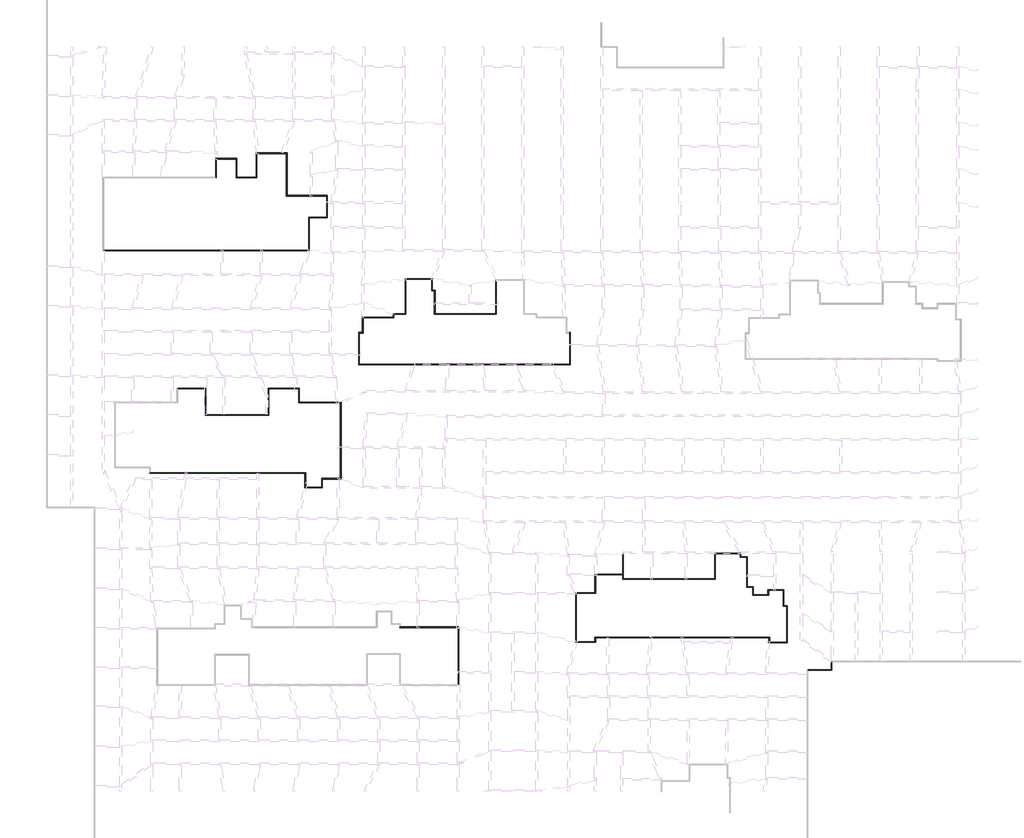
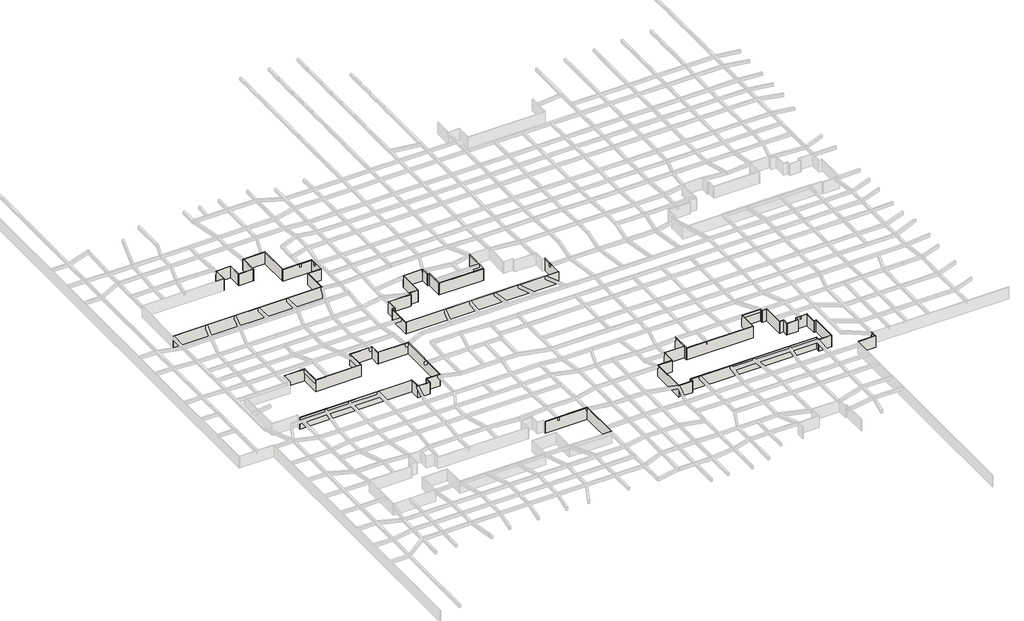
# One storey, part 3 of 45: 68 walls.
"""IFC4 building model written with IfcOpenShell, lengths in millimetres."""

from ifc_helpers import new_model, si_unit, origin, origin_with_axes, place, context, project, spatial, polyline, outline, extrude, faceted_brep, element, save

model = new_model("IFC4")

# Units and contexts
model_context = context("Model", 3, world=origin())
ifc_project = project(units=[si_unit("LENGTHUNIT", "METRE", prefix="MILLI")], contexts=[model_context])

# Site, building, storey
site = spatial("IfcSite", under=ifc_project)
building = spatial("IfcBuilding", under=site)
storey = spatial("IfcBuildingStorey", under=building, Name="户型图", Elevation=0.0)

# Walls
placement = place(None, origin())
element("IfcWall", 1, ObjectType="所有墙体", at=placement, inside=storey, context=model_context, shape_type="Brep", body=[
    faceted_brep([(-4880.5216564, -111688.0123265, 0.0), (-180.5216564, -111688.0123265, 0.0), (-180.5216564, -111688.0123265, 3300.0), (-4880.5216564, -111688.0123265, 3300.0), (-4880.5216564, -111568.0123265, 0.0), (-4880.5216564, -111568.0123265, 3300.0), (-300.5216564, -111568.0123265, 3300.0), (-180.5216564, -111568.0123265, 3300.0), (-180.5216564, -111568.0123265, 0.0), (-300.5216564, -111568.0123265, 0.0)], [[[0, 1, 2, 3]], [[4, 5, 6, 7, 8, 9]], [[1, 0, 4, 9, 8]], [[3, 2, 7, 6, 5]], [[0, 3, 5, 4]], [[2, 1, 8, 7]]]),
])
element("IfcWall", 2, ObjectType="所有墙体", at=placement, inside=storey, context=model_context, shape_type="Brep", body=[
    faceted_brep([(-180.5216564, -111568.0123265, 0.0), (-180.5216564, -109988.0123265, 0.0), (-180.5216564, -109868.0123265, 0.0), (-180.5216564, -109868.0123265, 3300.0), (-180.5216564, -109988.0123265, 3300.0), (-180.5216564, -111568.0123265, 3300.0), (-300.5216564, -111568.0123265, 0.0), (-300.5216564, -111568.0123265, 3300.0), (-300.5216564, -109868.0123265, 3300.0), (-300.5216564, -109868.0123265, 0.0)], [[[0, 1, 2, 3, 4, 5]], [[6, 7, 8, 9]], [[2, 1, 0, 6, 9]], [[5, 4, 3, 8, 7]], [[0, 5, 7, 6]], [[3, 2, 9, 8]]]),
])
element("IfcWall", 3, ObjectType="所有墙体", at=placement, inside=storey, context=model_context, shape_type="Brep", body=[
    faceted_brep([(-73790.9438267, -114496.2273817, 0.0), (-73790.9438267, -103096.2273817, 0.0), (-73790.9438267, -103096.2273817, 3300.0), (-73790.9438267, -114496.2273817, 3300.0), (-73910.9438267, -114496.2273817, 0.0), (-73910.9438267, -114496.2273817, 3300.0), (-73910.9438267, -103216.2273817, 3300.0), (-73910.9438267, -103096.2273817, 3300.0), (-73910.9438267, -103096.2273817, 0.0), (-73910.9438267, -103216.2273817, 0.0)], [[[0, 1, 2, 3]], [[4, 5, 6, 7, 8, 9]], [[1, 0, 4, 9, 8]], [[3, 2, 7, 6, 5]], [[0, 3, 5, 4]], [[2, 1, 8, 7]]]),
])
element("IfcWall", 4, ObjectType="所有墙体", at=placement, inside=storey, context=model_context, shape_type="Brep", body=[
    faceted_brep([(-73910.9438267, -103096.2273817, 0.0), (-85290.9438267, -103096.2273817, 0.0), (-85410.9438267, -103096.2273817, 0.0), (-85410.9438267, -103096.2273817, 3300.0), (-85290.9438267, -103096.2273817, 3300.0), (-73910.9438267, -103096.2273817, 3300.0), (-73910.9438267, -103216.2273817, 0.0), (-73910.9438267, -103216.2273817, 3300.0), (-85410.9438267, -103216.2273817, 3300.0), (-85410.9438267, -103216.2273817, 0.0)], [[[0, 1, 2, 3, 4, 5]], [[6, 7, 8, 9]], [[2, 1, 0, 6, 9]], [[5, 4, 3, 8, 7]], [[0, 5, 7, 6]], [[3, 2, 9, 8]]]),
])
element("IfcWall", 5, ObjectType="所有墙体", at=placement, inside=storey, context=model_context, shape_type="Brep", body=[
    faceted_brep([(-50591.7004294, -106142.3307416, 0.0), (-50591.7004294, -106022.3307416, 0.0), (-50591.7004294, -96442.3307416, 0.0), (-50591.7004294, -96322.3307416, 0.0), (-50591.7004294, -96322.3307416, 3300.0), (-50591.7004294, -96442.3307416, 3300.0), (-50591.7004294, -106022.3307416, 3300.0), (-50591.7004294, -106142.3307416, 3300.0), (-50711.7004294, -106142.3307416, 0.0), (-50711.7004294, -106142.3307416, 3300.0), (-50711.7004294, -96322.3307416, 3300.0), (-50711.7004294, -96322.3307416, 0.0)], [[[0, 1, 2, 3, 4, 5, 6, 7]], [[8, 9, 10, 11]], [[3, 2, 1, 0, 8, 11]], [[7, 6, 5, 4, 10, 9]], [[4, 3, 11, 10]], [[0, 7, 9, 8]]]),
])
element("IfcWall", 6, ObjectType="所有墙体", at=placement, inside=storey, context=model_context, shape_type="Brep", body=[
    faceted_brep([(-50591.7004294, -96442.3307416, 0.0), (-46791.7004294, -96442.3307416, 0.0), (-46791.7004294, -96442.3307416, 3300.0), (-50591.7004294, -96442.3307416, 3300.0), (-50591.7004294, -96322.3307416, 0.0), (-50591.7004294, -96322.3307416, 3300.0), (-46911.7004294, -96322.3307416, 3300.0), (-46791.7004294, -96322.3307416, 3300.0), (-46791.7004294, -96322.3307416, 0.0), (-46911.7004294, -96322.3307416, 0.0)], [[[0, 1, 2, 3]], [[4, 5, 6, 7, 8, 9]], [[1, 0, 4, 9, 8]], [[3, 2, 7, 6, 5]], [[0, 3, 5, 4]], [[2, 1, 8, 7]]]),
])
element("IfcWall", 7, ObjectType="所有墙体", at=placement, inside=storey, context=model_context, shape_type="Brep", body=[
    faceted_brep([(-46791.7004294, -96322.3307416, 0.0), (-46791.7004294, -92842.3307416, 0.0), (-46791.7004294, -92722.3307416, 0.0), (-46791.7004294, -92722.3307416, 3300.0), (-46791.7004294, -92842.3307416, 3300.0), (-46791.7004294, -96322.3307416, 3300.0), (-46911.7004294, -96322.3307416, 0.0), (-46911.7004294, -96322.3307416, 3300.0), (-46911.7004294, -92722.3307416, 3300.0), (-46911.7004294, -92722.3307416, 0.0)], [[[0, 1, 2, 3, 4, 5]], [[6, 7, 8, 9]], [[2, 1, 0, 6, 9]], [[5, 4, 3, 8, 7]], [[0, 5, 7, 6]], [[3, 2, 9, 8]]]),
])
element("IfcWall", 8, ObjectType="所有墙体", at=placement, inside=storey, context=model_context, shape_type="SweptSolid", body=[
    extrude(outline(polyline([(-41411.7004294, -92842.3307416), (-46791.7004294, -92842.3307416), (-46791.7004294, -92722.3307416), (-41411.7004294, -92722.3307416), (-41411.7004294, -92842.3307416)])), origin_with_axes(), (0.0, 0.0, 1.0), 3300.0),
])
element("IfcWall", 9, ObjectType="所有墙体", at=placement, inside=storey, context=model_context, shape_type="Brep", body=[
    faceted_brep([(-41291.7004294, -93742.3307416, 0.0), (-41291.7004294, -93622.3307416, 0.0), (-41291.7004294, -88582.3307416, 0.0), (-41291.7004294, -88582.3307416, 3300.0), (-41291.7004294, -93622.3307416, 3300.0), (-41291.7004294, -93742.3307416, 3300.0), (-41411.7004294, -93742.3307416, 0.0), (-41411.7004294, -93742.3307416, 3300.0), (-41411.7004294, -92842.3307416, 3300.0), (-41411.7004294, -92722.3307416, 3300.0), (-41411.7004294, -88582.3307416, 3300.0), (-41411.7004294, -88582.3307416, 0.0), (-41411.7004294, -92722.3307416, 0.0), (-41411.7004294, -92842.3307416, 0.0)], [[[0, 1, 2, 3, 4, 5]], [[6, 7, 8, 9, 10, 11, 12, 13]], [[2, 1, 0, 6, 13, 12, 11]], [[3, 2, 11, 10]], [[5, 4, 3, 10, 9, 8, 7]], [[0, 5, 7, 6]]]),
])
element("IfcWall", 10, ObjectType="所有墙体", at=placement, inside=storey, context=model_context, shape_type="Brep", body=[
    faceted_brep([(-41291.7004294, -93742.3307416, 0.0), (-23191.7004294, -93742.3307416, 0.0), (-23191.7004294, -93742.3307416, 3300.0), (-41291.7004294, -93742.3307416, 3300.0), (-41291.7004294, -93622.3307416, 0.0), (-41291.7004294, -93622.3307416, 3300.0), (-23311.7004294, -93622.3307416, 3300.0), (-23191.7004294, -93622.3307416, 3300.0), (-23191.7004294, -93622.3307416, 0.0), (-23311.7004294, -93622.3307416, 0.0)], [[[0, 1, 2, 3]], [[4, 5, 6, 7, 8, 9]], [[1, 0, 4, 9, 8]], [[3, 2, 7, 6, 5]], [[0, 3, 5, 4]], [[2, 1, 8, 7]]]),
])
element("IfcWall", 11, ObjectType="所有墙体", at=placement, inside=storey, context=model_context, shape_type="Brep", body=[
    faceted_brep([(-23191.7004294, -93622.3307416, 0.0), (-23191.7004294, -88647.9389906, 0.0), (-23191.7004294, -88527.9389906, 0.0), (-23191.7004294, -88527.9389906, 3300.0), (-23191.7004294, -88647.9389906, 3300.0), (-23191.7004294, -93622.3307416, 3300.0), (-23311.7004294, -93622.3307416, 0.0), (-23311.7004294, -93622.3307416, 3300.0), (-23311.7004294, -88527.9389906, 3300.0), (-23311.7004294, -88527.9389906, 0.0)], [[[0, 1, 2, 3, 4, 5]], [[6, 7, 8, 9]], [[2, 1, 0, 6, 9]], [[5, 4, 3, 8, 7]], [[0, 5, 7, 6]], [[3, 2, 9, 8]]]),
])
element("IfcWall", 12, ObjectType="所有墙体", at=placement, inside=storey, context=model_context, shape_type="Brep", body=[
    faceted_brep([(-23191.7004294, -88647.9389906, 0.0), (-18278.6749736, -88647.9389906, 0.0), (-18158.6749736, -88647.9389906, 0.0), (-18158.6749736, -88647.9389906, 3300.0), (-18278.6749736, -88647.9389906, 3300.0), (-23191.7004294, -88647.9389906, 3300.0), (-23191.7004294, -88527.9389906, 0.0), (-23191.7004294, -88527.9389906, 3300.0), (-18158.6749736, -88527.9389906, 3300.0), (-18158.6749736, -88527.9389906, 0.0)], [[[0, 1, 2, 3, 4, 5]], [[6, 7, 8, 9]], [[2, 1, 0, 6, 9]], [[5, 4, 3, 8, 7]], [[0, 5, 7, 6]], [[3, 2, 9, 8]]]),
])
element("IfcWall", 13, ObjectType="所有墙体", at=placement, inside=storey, context=model_context, shape_type="Brep", body=[
    faceted_brep([(-16858.6749736, -95247.9389906, 0.0), (-15778.6749736, -95247.9389906, 0.0), (-15658.6749736, -95247.9389906, 0.0), (-15658.6749736, -95247.9389906, 3300.0), (-15778.6749736, -95247.9389906, 3300.0), (-16858.6749736, -95247.9389906, 3300.0), (-16858.6749736, -95127.9389906, 0.0), (-16858.6749736, -95127.9389906, 3300.0), (-15658.6749736, -95127.9389906, 3300.0), (-15658.6749736, -95127.9389906, 0.0)], [[[0, 1, 2, 3, 4, 5]], [[6, 7, 8, 9]], [[2, 1, 0, 6, 9]], [[5, 4, 3, 8, 7]], [[3, 2, 9, 8]], [[0, 5, 7, 6]]]),
])
element("IfcWall", 14, ObjectType="所有墙体", at=placement, inside=storey, context=model_context, shape_type="Brep", body=[
    faceted_brep([(-15778.6749736, -95247.9389906, 0.0), (-15778.6749736, -96847.9389906, 0.0), (-15778.6749736, -96847.9389906, 3300.0), (-15778.6749736, -95247.9389906, 3300.0), (-15658.6749736, -95247.9389906, 0.0), (-15658.6749736, -95247.9389906, 3300.0), (-15658.6749736, -96727.9389906, 3300.0), (-15658.6749736, -96847.9389906, 3300.0), (-15658.6749736, -96847.9389906, 0.0), (-15658.6749736, -96727.9389906, 0.0)], [[[0, 1, 2, 3]], [[4, 5, 6, 7, 8, 9]], [[1, 0, 4, 9, 8]], [[3, 2, 7, 6, 5]], [[0, 3, 5, 4]], [[2, 1, 8, 7]]]),
])
element("IfcWall", 15, ObjectType="所有墙体", at=placement, inside=storey, context=model_context, shape_type="Brep", body=[
    faceted_brep([(-15658.6749736, -96847.9389906, 0.0), (-12658.6749736, -96847.9389906, 0.0), (-12658.6749736, -96847.9389906, 3300.0), (-15658.6749736, -96847.9389906, 3300.0), (-15658.6749736, -96727.9389906, 0.0), (-15658.6749736, -96727.9389906, 3300.0), (-12778.6749736, -96727.9389906, 3300.0), (-12658.6749736, -96727.9389906, 3300.0), (-12658.6749736, -96727.9389906, 0.0), (-12778.6749736, -96727.9389906, 0.0)], [[[0, 1, 2, 3]], [[4, 5, 6, 7, 8, 9]], [[1, 0, 4, 9, 8]], [[3, 2, 7, 6, 5]], [[0, 3, 5, 4]], [[2, 1, 8, 7]]]),
])
element("IfcWall", 16, ObjectType="所有墙体", at=placement, inside=storey, context=model_context, shape_type="Brep", body=[
    faceted_brep([(-12658.6749736, -96727.9389906, 0.0), (-12658.6749736, -95847.9389906, 0.0), (-12658.6749736, -95727.9389906, 0.0), (-12658.6749736, -95727.9389906, 3300.0), (-12658.6749736, -95847.9389906, 3300.0), (-12658.6749736, -96727.9389906, 3300.0), (-12778.6749736, -96727.9389906, 0.0), (-12778.6749736, -96727.9389906, 3300.0), (-12778.6749736, -95727.9389906, 3300.0), (-12778.6749736, -95727.9389906, 0.0)], [[[0, 1, 2, 3, 4, 5]], [[6, 7, 8, 9]], [[2, 1, 0, 6, 9]], [[5, 4, 3, 8, 7]], [[0, 5, 7, 6]], [[3, 2, 9, 8]]]),
])
element("IfcWall", 17, ObjectType="所有墙体", at=placement, inside=storey, context=model_context, shape_type="Brep", body=[
    faceted_brep([(-12658.6749736, -95847.9389906, 0.0), (-9778.6749736, -95847.9389906, 0.0), (-9658.6749736, -95847.9389906, 0.0), (-9658.6749736, -95847.9389906, 3300.0), (-9778.6749736, -95847.9389906, 3300.0), (-12658.6749736, -95847.9389906, 3300.0), (-12658.6749736, -95727.9389906, 0.0), (-12658.6749736, -95727.9389906, 3300.0), (-9658.6749736, -95727.9389906, 3300.0), (-9658.6749736, -95727.9389906, 0.0)], [[[0, 1, 2, 3, 4, 5]], [[6, 7, 8, 9]], [[2, 1, 0, 6, 9]], [[5, 4, 3, 8, 7]], [[0, 5, 7, 6]], [[3, 2, 9, 8]]]),
])
element("IfcWall", 18, ObjectType="所有墙体", at=placement, inside=storey, context=model_context, shape_type="Brep", body=[
    faceted_brep([(-9778.6749736, -95847.9389906, 0.0), (-9778.6749736, -99047.9389906, 0.0), (-9778.6749736, -99047.9389906, 3300.0), (-9778.6749736, -95847.9389906, 3300.0), (-9658.6749736, -95847.9389906, 0.0), (-9658.6749736, -95847.9389906, 3300.0), (-9658.6749736, -98927.9389906, 3300.0), (-9658.6749736, -99047.9389906, 3300.0), (-9658.6749736, -99047.9389906, 0.0), (-9658.6749736, -98927.9389906, 0.0)], [[[0, 1, 2, 3]], [[4, 5, 6, 7, 8, 9]], [[1, 0, 4, 9, 8]], [[3, 2, 7, 6, 5]], [[0, 3, 5, 4]], [[2, 1, 8, 7]]]),
])
element("IfcWall", 19, ObjectType="所有墙体", at=placement, inside=storey, context=model_context, shape_type="Brep", body=[
    faceted_brep([(-9658.6749736, -99047.9389906, 0.0), (-9078.6749736, -99047.9389906, 0.0), (-8958.6749736, -99047.9389906, 0.0), (-8958.6749736, -99047.9389906, 3300.0), (-9078.6749736, -99047.9389906, 3300.0), (-9658.6749736, -99047.9389906, 3300.0), (-9658.6749736, -98927.9389906, 0.0), (-9658.6749736, -98927.9389906, 3300.0), (-8958.6749736, -98927.9389906, 3300.0), (-8958.6749736, -98927.9389906, 0.0)], [[[0, 1, 2, 3, 4, 5]], [[6, 7, 8, 9]], [[2, 1, 0, 6, 9]], [[5, 4, 3, 8, 7]], [[0, 5, 7, 6]], [[3, 2, 9, 8]]]),
])
element("IfcWall", 20, ObjectType="所有墙体", at=placement, inside=storey, context=model_context, shape_type="Brep", body=[
    faceted_brep([(-9078.6749736, -99047.9389906, 0.0), (-9078.6749736, -106127.9389906, 0.0), (-9078.6749736, -106247.9389906, 0.0), (-9078.6749736, -106247.9389906, 3300.0), (-9078.6749736, -106127.9389906, 3300.0), (-9078.6749736, -99047.9389906, 3300.0), (-8958.6749736, -99047.9389906, 0.0), (-8958.6749736, -99047.9389906, 3300.0), (-8958.6749736, -106247.9389906, 3300.0), (-8958.6749736, -106247.9389906, 0.0)], [[[0, 1, 2, 3, 4, 5]], [[6, 7, 8, 9]], [[2, 1, 0, 6, 9]], [[5, 4, 3, 8, 7]], [[0, 5, 7, 6]], [[3, 2, 9, 8]]]),
])
element("IfcWall", 21, ObjectType="所有墙体", at=placement, inside=storey, context=model_context, shape_type="Brep", body=[
    faceted_brep([(-9078.6749736, -106127.9389906, 0.0), (-12457.3241974, -106127.9389906, 0.0), (-12577.3241974, -106127.9389906, 0.0), (-12577.3241974, -106127.9389906, 3300.0), (-12457.3241974, -106127.9389906, 3300.0), (-9078.6749736, -106127.9389906, 3300.0), (-9078.6749736, -106247.9389906, 0.0), (-9078.6749736, -106247.9389906, 3300.0), (-12577.3241974, -106247.9389906, 3300.0), (-12577.3241974, -106247.9389906, 0.0)], [[[0, 1, 2, 3, 4, 5]], [[6, 7, 8, 9]], [[2, 1, 0, 6, 9]], [[5, 4, 3, 8, 7]], [[0, 5, 7, 6]], [[3, 2, 9, 8]]]),
])
element("IfcWall", 22, ObjectType="所有墙体", at=placement, inside=storey, context=model_context, shape_type="Brep", body=[
    faceted_brep([(-12457.3241974, -106127.9389906, 0.0), (-12457.3241974, -105127.9389906, 0.0), (-12457.3241974, -105127.9389906, 3300.0), (-12457.3241974, -106127.9389906, 3300.0), (-12577.3241974, -106127.9389906, 0.0), (-12577.3241974, -106127.9389906, 3300.0), (-12577.3241974, -105247.9389906, 3300.0), (-12577.3241974, -105127.9389906, 3300.0), (-12577.3241974, -105127.9389906, 0.0), (-12577.3241974, -105247.9389906, 0.0)], [[[0, 1, 2, 3]], [[4, 5, 6, 7, 8, 9]], [[1, 0, 4, 9, 8]], [[3, 2, 7, 6, 5]], [[0, 3, 5, 4]], [[2, 1, 8, 7]]]),
])
element("IfcWall", 23, ObjectType="所有墙体", at=placement, inside=storey, context=model_context, shape_type="Brep", body=[
    faceted_brep([(-12577.3241974, -105127.9389906, 0.0), (-46911.7004294, -105127.9389906, 0.0), (-46911.7004294, -105127.9389906, 3300.0), (-12577.3241974, -105127.9389906, 3300.0), (-12577.3241974, -105247.9389906, 0.0), (-12577.3241974, -105247.9389906, 3300.0), (-46791.7004294, -105247.9389906, 3300.0), (-46911.7004294, -105247.9389906, 3300.0), (-46911.7004294, -105247.9389906, 0.0), (-46791.7004294, -105247.9389906, 0.0)], [[[0, 1, 2, 3]], [[4, 5, 6, 7, 8, 9]], [[1, 0, 4, 9, 8]], [[3, 2, 7, 6, 5]], [[0, 3, 5, 4]], [[2, 1, 8, 7]]]),
])
element("IfcWall", 24, ObjectType="所有墙体", at=placement, inside=storey, context=model_context, shape_type="Brep", body=[
    faceted_brep([(-46911.7004294, -105247.9389906, 0.0), (-46911.7004294, -106022.3307416, 0.0), (-46911.7004294, -106142.3307416, 0.0), (-46911.7004294, -106142.3307416, 3300.0), (-46911.7004294, -106022.3307416, 3300.0), (-46911.7004294, -105247.9389906, 3300.0), (-46791.7004294, -105247.9389906, 0.0), (-46791.7004294, -105247.9389906, 3300.0), (-46791.7004294, -106142.3307416, 3300.0), (-46791.7004294, -106142.3307416, 0.0)], [[[0, 1, 2, 3, 4, 5]], [[6, 7, 8, 9]], [[2, 1, 0, 6, 9]], [[5, 4, 3, 8, 7]], [[0, 5, 7, 6]], [[3, 2, 9, 8]]]),
])
element("IfcWall", 25, ObjectType="所有墙体", at=placement, inside=storey, context=model_context, shape_type="SweptSolid", body=[
    extrude(outline(polyline([(-50591.7004294, -106022.3307416), (-46911.7004294, -106022.3307416), (-46911.7004294, -106142.3307416), (-50591.7004294, -106142.3307416), (-50591.7004294, -106022.3307416)])), origin_with_axes(), (0.0, 0.0, 1.0), 3300.0),
])
element("IfcWall", 26, ObjectType="所有墙体", at=placement, inside=storey, context=model_context, shape_type="Brep", body=[
    faceted_brep([(-18278.6749736, -88647.9389906, 0.0), (-18278.6749736, -89347.9389906, 0.0), (-18278.6749736, -89347.9389906, 3300.0), (-18278.6749736, -88647.9389906, 3300.0), (-18158.6749736, -88647.9389906, 0.0), (-18158.6749736, -88647.9389906, 3300.0), (-18158.6749736, -89227.9389906, 3300.0), (-18158.6749736, -89347.9389906, 3300.0), (-18158.6749736, -89347.9389906, 0.0), (-18158.6749736, -89227.9389906, 0.0)], [[[0, 1, 2, 3]], [[4, 5, 6, 7, 8, 9]], [[1, 0, 4, 9, 8]], [[3, 2, 7, 6, 5]], [[0, 3, 5, 4]], [[2, 1, 8, 7]]]),
])
element("IfcWall", 27, ObjectType="所有墙体", at=placement, inside=storey, context=model_context, shape_type="Brep", body=[
    faceted_brep([(-18158.6749736, -89347.9389906, 0.0), (-16978.6749736, -89347.9389906, 0.0), (-16858.6749736, -89347.9389906, 0.0), (-16858.6749736, -89347.9389906, 3300.0), (-16978.6749736, -89347.9389906, 3300.0), (-18158.6749736, -89347.9389906, 3300.0), (-18158.6749736, -89227.9389906, 0.0), (-18158.6749736, -89227.9389906, 3300.0), (-16858.6749736, -89227.9389906, 3300.0), (-16858.6749736, -89227.9389906, 0.0)], [[[0, 1, 2, 3, 4, 5]], [[6, 7, 8, 9]], [[2, 1, 0, 6, 9]], [[5, 4, 3, 8, 7]], [[0, 5, 7, 6]], [[3, 2, 9, 8]]]),
])
element("IfcWall", 28, ObjectType="所有墙体", at=placement, inside=storey, context=model_context, shape_type="Brep", body=[
    faceted_brep([(-16978.6749736, -89347.9389906, 0.0), (-16978.6749736, -95247.9389906, 0.0), (-16978.6749736, -95247.9389906, 3300.0), (-16978.6749736, -89347.9389906, 3300.0), (-16858.6749736, -89347.9389906, 0.0), (-16858.6749736, -89347.9389906, 3300.0), (-16858.6749736, -95127.9389906, 3300.0), (-16858.6749736, -95247.9389906, 3300.0), (-16858.6749736, -95247.9389906, 0.0), (-16858.6749736, -95127.9389906, 0.0)], [[[0, 1, 2, 3]], [[4, 5, 6, 7, 8, 9]], [[1, 0, 4, 9, 8]], [[3, 2, 7, 6, 5]], [[0, 3, 5, 4]], [[2, 1, 8, 7]]]),
])
element("IfcWall", 29, ObjectType="所有墙体", at=placement, inside=storey, context=model_context, shape_type="Brep", body=[
    faceted_brep([(-129248.6297755, -56149.4871623, 0.0), (-123786.6222431, -56149.4871623, 0.0), (-123666.6222431, -56149.4871623, 0.0), (-123666.6222431, -56149.4871623, 3300.0), (-123786.6222431, -56149.4871623, 3300.0), (-129248.6297755, -56149.4871623, 3300.0), (-129248.6297755, -56029.4871623, 0.0), (-129248.6297755, -56029.4871623, 3300.0), (-123666.6222431, -56029.4871623, 3300.0), (-123666.6222431, -56029.4871623, 0.0)], [[[0, 1, 2, 3, 4, 5]], [[6, 7, 8, 9]], [[2, 1, 0, 6, 9]], [[5, 4, 3, 8, 7]], [[0, 5, 7, 6]], [[3, 2, 9, 8]]]),
])
element("IfcWall", 30, ObjectType="所有墙体", at=placement, inside=storey, context=model_context, shape_type="Brep", body=[
    faceted_brep([(-123786.6222431, -56149.4871623, 0.0), (-123786.6222431, -61349.4871623, 0.0), (-123786.6222431, -61349.4871623, 3300.0), (-123786.6222431, -56149.4871623, 3300.0), (-123666.6222431, -56149.4871623, 0.0), (-123666.6222431, -56149.4871623, 3300.0), (-123666.6222431, -61229.4871623, 3300.0), (-123666.6222431, -61349.4871623, 3300.0), (-123666.6222431, -61349.4871623, 0.0), (-123666.6222431, -61229.4871623, 0.0)], [[[0, 1, 2, 3]], [[4, 5, 6, 7, 8, 9]], [[1, 0, 4, 9, 8]], [[3, 2, 7, 6, 5]], [[0, 3, 5, 4]], [[2, 1, 8, 7]]]),
])
element("IfcWall", 31, ObjectType="所有墙体", at=placement, inside=storey, context=model_context, shape_type="Brep", body=[
    faceted_brep([(-123666.6222431, -61349.4871623, 0.0), (-111266.6222431, -61349.4871623, 0.0), (-111266.6222431, -61349.4871623, 3300.0), (-123666.6222431, -61349.4871623, 3300.0), (-123666.6222431, -61229.4871623, 0.0), (-123666.6222431, -61229.4871623, 3300.0), (-111386.6222431, -61229.4871623, 3300.0), (-111266.6222431, -61229.4871623, 3300.0), (-111266.6222431, -61229.4871623, 0.0), (-111386.6222431, -61229.4871623, 0.0)], [[[0, 1, 2, 3]], [[4, 5, 6, 7, 8, 9]], [[1, 0, 4, 9, 8]], [[3, 2, 7, 6, 5]], [[0, 3, 5, 4]], [[2, 1, 8, 7]]]),
])
element("IfcWall", 32, ObjectType="所有墙体", at=placement, inside=storey, context=model_context, shape_type="Brep", body=[
    faceted_brep([(-111266.6222431, -61229.4871623, 0.0), (-111266.6222431, -56149.4871623, 0.0), (-111266.6222431, -56029.4871623, 0.0), (-111266.6222431, -56029.4871623, 3300.0), (-111266.6222431, -56149.4871623, 3300.0), (-111266.6222431, -61229.4871623, 3300.0), (-111386.6222431, -61229.4871623, 0.0), (-111386.6222431, -61229.4871623, 3300.0), (-111386.6222431, -56029.4871623, 3300.0), (-111386.6222431, -56029.4871623, 0.0)], [[[0, 1, 2, 3, 4, 5]], [[6, 7, 8, 9]], [[2, 1, 0, 6, 9]], [[5, 4, 3, 8, 7]], [[0, 5, 7, 6]], [[3, 2, 9, 8]]]),
])
element("IfcWall", 33, ObjectType="所有墙体", at=placement, inside=storey, context=model_context, shape_type="Brep", body=[
    faceted_brep([(-111266.6222431, -56149.4871623, 0.0), (-105386.6222431, -56149.4871623, 0.0), (-105266.6222431, -56149.4871623, 0.0), (-105266.6222431, -56149.4871623, 3300.0), (-105386.6222431, -56149.4871623, 3300.0), (-111266.6222431, -56149.4871623, 3300.0), (-111266.6222431, -56029.4871623, 0.0), (-111266.6222431, -56029.4871623, 3300.0), (-105266.6222431, -56029.4871623, 3300.0), (-105266.6222431, -56029.4871623, 0.0)], [[[0, 1, 2, 3, 4, 5]], [[6, 7, 8, 9]], [[2, 1, 0, 6, 9]], [[5, 4, 3, 8, 7]], [[0, 5, 7, 6]], [[3, 2, 9, 8]]]),
])
element("IfcWall", 34, ObjectType="所有墙体", at=placement, inside=storey, context=model_context, shape_type="Brep", body=[
    faceted_brep([(-105386.6222431, -56149.4871623, 0.0), (-105386.6222431, -58849.4871623, 0.0), (-105386.6222431, -58849.4871623, 3300.0), (-105386.6222431, -56149.4871623, 3300.0), (-105266.6222431, -56149.4871623, 0.0), (-105266.6222431, -56149.4871623, 3300.0), (-105266.6222431, -58729.4871623, 3300.0), (-105266.6222431, -58849.4871623, 3300.0), (-105266.6222431, -58849.4871623, 0.0), (-105266.6222431, -58729.4871623, 0.0)], [[[0, 1, 2, 3]], [[4, 5, 6, 7, 8, 9]], [[1, 0, 4, 9, 8]], [[3, 2, 7, 6, 5]], [[0, 3, 5, 4]], [[2, 1, 8, 7]]]),
])
element("IfcWall", 35, ObjectType="所有墙体", at=placement, inside=storey, context=model_context, shape_type="Brep", body=[
    faceted_brep([(-105266.6222431, -58849.4871623, 0.0), (-97113.3068729, -58849.4871623, 0.0), (-96993.3068729, -58849.4871623, 0.0), (-96993.3068729, -58849.4871623, 3300.0), (-97113.3068729, -58849.4871623, 3300.0), (-105266.6222431, -58849.4871623, 3300.0), (-105266.6222431, -58729.4871623, 0.0), (-105266.6222431, -58729.4871623, 3300.0), (-96993.3068729, -58729.4871623, 3300.0), (-96993.3068729, -58729.4871623, 0.0)], [[[0, 1, 2, 3, 4, 5]], [[6, 7, 8, 9]], [[2, 1, 0, 6, 9]], [[5, 4, 3, 8, 7]], [[0, 5, 7, 6]], [[3, 2, 9, 8]]]),
])
element("IfcWall", 36, ObjectType="所有墙体", at=placement, inside=storey, context=model_context, shape_type="Brep", body=[
    faceted_brep([(-97113.3068729, -58849.4871623, 0.0), (-97113.3068729, -73798.7850558, 0.0), (-97113.3068729, -73918.7850558, 0.0), (-97113.3068729, -73918.7850558, 3300.0), (-97113.3068729, -73798.7850558, 3300.0), (-97113.3068729, -58849.4871623, 3300.0), (-96993.3068729, -58849.4871623, 0.0), (-96993.3068729, -58849.4871623, 3300.0), (-96993.3068729, -73918.7850558, 3300.0), (-96993.3068729, -73918.7850558, 0.0)], [[[0, 1, 2, 3, 4, 5]], [[6, 7, 8, 9]], [[2, 1, 0, 6, 9]], [[5, 4, 3, 8, 7]], [[0, 5, 7, 6]], [[3, 2, 9, 8]]]),
])
element("IfcWall", 37, ObjectType="所有墙体", at=placement, inside=storey, context=model_context, shape_type="Brep", body=[
    faceted_brep([(-97113.3068729, -73798.7850558, 0.0), (-100813.3068729, -73798.7850558, 0.0), (-100813.3068729, -73798.7850558, 3300.0), (-97113.3068729, -73798.7850558, 3300.0), (-97113.3068729, -73918.7850558, 0.0), (-97113.3068729, -73918.7850558, 3300.0), (-100693.3068729, -73918.7850558, 3300.0), (-100813.3068729, -73918.7850558, 3300.0), (-100813.3068729, -73918.7850558, 0.0), (-100693.3068729, -73918.7850558, 0.0)], [[[0, 1, 2, 3]], [[4, 5, 6, 7, 8, 9]], [[1, 0, 4, 9, 8]], [[3, 2, 7, 6, 5]], [[0, 3, 5, 4]], [[2, 1, 8, 7]]]),
])
element("IfcWall", 38, ObjectType="所有墙体", at=placement, inside=storey, context=model_context, shape_type="Brep", body=[
    faceted_brep([(-100813.3068729, -73918.7850558, 0.0), (-100813.3068729, -75498.7850558, 0.0), (-100813.3068729, -75618.7850558, 0.0), (-100813.3068729, -75618.7850558, 3300.0), (-100813.3068729, -75498.7850558, 3300.0), (-100813.3068729, -73918.7850558, 3300.0), (-100693.3068729, -73918.7850558, 0.0), (-100693.3068729, -73918.7850558, 3300.0), (-100693.3068729, -75618.7850558, 3300.0), (-100693.3068729, -75618.7850558, 0.0)], [[[0, 1, 2, 3, 4, 5]], [[6, 7, 8, 9]], [[2, 1, 0, 6, 9]], [[5, 4, 3, 8, 7]], [[0, 5, 7, 6]], [[3, 2, 9, 8]]]),
])
element("IfcWall", 39, ObjectType="所有墙体", at=placement, inside=storey, context=model_context, shape_type="Brep", body=[
    faceted_brep([(-100813.3068729, -75498.7850558, 0.0), (-104004.8033987, -75498.7850558, 0.0), (-104124.8033987, -75498.7850558, 0.0), (-104124.8033987, -75498.7850558, 3300.0), (-104004.8033987, -75498.7850558, 3300.0), (-100813.3068729, -75498.7850558, 3300.0), (-100813.3068729, -75618.7850558, 0.0), (-100813.3068729, -75618.7850558, 3300.0), (-104124.8033987, -75618.7850558, 3300.0), (-104124.8033987, -75618.7850558, 0.0)], [[[0, 1, 2, 3, 4, 5]], [[6, 7, 8, 9]], [[2, 1, 0, 6, 9]], [[5, 4, 3, 8, 7]], [[0, 5, 7, 6]], [[3, 2, 9, 8]]]),
])
element("IfcWall", 40, ObjectType="所有墙体", at=placement, inside=storey, context=model_context, shape_type="Brep", body=[
    faceted_brep([(-104004.8033987, -75498.7850558, 0.0), (-104004.8033987, -72698.7850558, 0.0), (-104004.8033987, -72698.7850558, 3300.0), (-104004.8033987, -75498.7850558, 3300.0), (-104124.8033987, -75498.7850558, 0.0), (-104124.8033987, -75498.7850558, 3300.0), (-104124.8033987, -72818.7850558, 3300.0), (-104124.8033987, -72698.7850558, 3300.0), (-104124.8033987, -72698.7850558, 0.0), (-104124.8033987, -72818.7850558, 0.0)], [[[0, 1, 2, 3]], [[4, 5, 6, 7, 8, 9]], [[1, 0, 4, 9, 8]], [[3, 2, 7, 6, 5]], [[0, 3, 5, 4]], [[2, 1, 8, 7]]]),
])
element("IfcWall", 41, ObjectType="所有墙体", at=placement, inside=storey, context=model_context, shape_type="Brep", body=[
    faceted_brep([(-104124.8033987, -72698.7850558, 0.0), (-134604.8033987, -72698.7850558, 0.0), (-134724.8033987, -72698.7850558, 0.0), (-134724.8033987, -72698.7850558, 3300.0), (-134604.8033987, -72698.7850558, 3300.0), (-104124.8033987, -72698.7850558, 3300.0), (-104124.8033987, -72818.7850558, 0.0), (-104124.8033987, -72818.7850558, 3300.0), (-134724.8033987, -72818.7850558, 3300.0), (-134724.8033987, -72818.7850558, 0.0)], [[[0, 1, 2, 3, 4, 5]], [[6, 7, 8, 9]], [[2, 1, 0, 6, 9]], [[5, 4, 3, 8, 7]], [[0, 5, 7, 6]], [[3, 2, 9, 8]]]),
])
element("IfcWall", 42, ObjectType="所有墙体", at=placement, inside=storey, context=model_context, shape_type="Brep", body=[
    faceted_brep([(-143844.0852782, -28883.8680223, 0.0), (-103244.0852782, -28883.8680223, 0.0), (-103244.0852782, -28883.8680223, 3300.0), (-143844.0852782, -28883.8680223, 3300.0), (-143844.0852782, -28763.8680223, 0.0), (-143844.0852782, -28763.8680223, 3300.0), (-103364.0852782, -28763.8680223, 3300.0), (-103244.0852782, -28763.8680223, 3300.0), (-103244.0852782, -28763.8680223, 0.0), (-103364.0852782, -28763.8680223, 0.0)], [[[0, 1, 2, 3]], [[4, 5, 6, 7, 8, 9]], [[1, 0, 4, 9, 8]], [[3, 2, 7, 6, 5]], [[0, 3, 5, 4]], [[2, 1, 8, 7]]]),
])
element("IfcWall", 43, ObjectType="所有墙体", at=placement, inside=storey, context=model_context, shape_type="Brep", body=[
    faceted_brep([(-103244.0852782, -28763.8680223, 0.0), (-103244.0852782, -22403.8680223, 0.0), (-103244.0852782, -22283.8680223, 0.0), (-103244.0852782, -22283.8680223, 3300.0), (-103244.0852782, -22403.8680223, 3300.0), (-103244.0852782, -28763.8680223, 3300.0), (-103364.0852782, -28763.8680223, 0.0), (-103364.0852782, -28763.8680223, 3300.0), (-103364.0852782, -22283.8680223, 3300.0), (-103364.0852782, -22283.8680223, 0.0)], [[[0, 1, 2, 3, 4, 5]], [[6, 7, 8, 9]], [[2, 1, 0, 6, 9]], [[5, 4, 3, 8, 7]], [[0, 5, 7, 6]], [[3, 2, 9, 8]]]),
])
element("IfcWall", 44, ObjectType="所有墙体", at=placement, inside=storey, context=model_context, shape_type="Brep", body=[
    faceted_brep([(-103244.0852782, -22403.8680223, 0.0), (-99744.0852782, -22403.8680223, 0.0), (-99744.0852782, -22403.8680223, 3300.0), (-103244.0852782, -22403.8680223, 3300.0), (-103244.0852782, -22283.8680223, 0.0), (-103244.0852782, -22283.8680223, 3300.0), (-99864.0852782, -22283.8680223, 3300.0), (-99744.0852782, -22283.8680223, 3300.0), (-99744.0852782, -22283.8680223, 0.0), (-99864.0852782, -22283.8680223, 0.0)], [[[0, 1, 2, 3]], [[4, 5, 6, 7, 8, 9]], [[1, 0, 4, 9, 8]], [[3, 2, 7, 6, 5]], [[0, 3, 5, 4]], [[2, 1, 8, 7]]]),
])
element("IfcWall", 45, ObjectType="所有墙体", at=placement, inside=storey, context=model_context, shape_type="Brep", body=[
    faceted_brep([(-99744.0852782, -22283.8680223, 0.0), (-99744.0852782, -17983.8680223, 0.0), (-99744.0852782, -17983.8680223, 3300.0), (-99744.0852782, -22283.8680223, 3300.0), (-99864.0852782, -22283.8680223, 0.0), (-99864.0852782, -22283.8680223, 3300.0), (-99864.0852782, -18103.8680223, 3300.0), (-99864.0852782, -17983.8680223, 3300.0), (-99864.0852782, -17983.8680223, 0.0), (-99864.0852782, -18103.8680223, 0.0)], [[[0, 1, 2, 3]], [[4, 5, 6, 7, 8, 9]], [[1, 0, 4, 9, 8]], [[3, 2, 7, 6, 5]], [[0, 3, 5, 4]], [[2, 1, 8, 7]]]),
])
element("IfcWall", 46, ObjectType="所有墙体", at=placement, inside=storey, context=model_context, shape_type="Brep", body=[
    faceted_brep([(-99864.0852782, -17983.8680223, 0.0), (-107644.0852782, -17983.8680223, 0.0), (-107764.0852782, -17983.8680223, 0.0), (-107764.0852782, -17983.8680223, 3300.0), (-107644.0852782, -17983.8680223, 3300.0), (-99864.0852782, -17983.8680223, 3300.0), (-99864.0852782, -18103.8680223, 0.0), (-99864.0852782, -18103.8680223, 3300.0), (-107764.0852782, -18103.8680223, 3300.0), (-107764.0852782, -18103.8680223, 0.0)], [[[0, 1, 2, 3, 4, 5]], [[6, 7, 8, 9]], [[2, 1, 0, 6, 9]], [[5, 4, 3, 8, 7]], [[0, 5, 7, 6]], [[3, 2, 9, 8]]]),
])
element("IfcWall", 47, ObjectType="所有墙体", at=placement, inside=storey, context=model_context, shape_type="Brep", body=[
    faceted_brep([(-107644.0852782, -17983.8680223, 0.0), (-107644.0852782, -9583.8680223, 0.0), (-107644.0852782, -9583.8680223, 3300.0), (-107644.0852782, -17983.8680223, 3300.0), (-107764.0852782, -17983.8680223, 0.0), (-107764.0852782, -17983.8680223, 3300.0), (-107764.0852782, -9703.8680223, 3300.0), (-107764.0852782, -9583.8680223, 3300.0), (-107764.0852782, -9583.8680223, 0.0), (-107764.0852782, -9703.8680223, 0.0)], [[[0, 1, 2, 3]], [[4, 5, 6, 7, 8, 9]], [[1, 0, 4, 9, 8]], [[3, 2, 7, 6, 5]], [[0, 3, 5, 4]], [[2, 1, 8, 7]]]),
])
element("IfcWall", 48, ObjectType="所有墙体", at=placement, inside=storey, context=model_context, shape_type="Brep", body=[
    faceted_brep([(-107764.0852782, -9583.8680223, 0.0), (-113717.1611319, -9583.8680223, 0.0), (-113717.1611319, -9583.8680223, 3300.0), (-107764.0852782, -9583.8680223, 3300.0), (-107764.0852782, -9703.8680223, 0.0), (-107764.0852782, -9703.8680223, 3300.0), (-113597.1611319, -9703.8680223, 3300.0), (-113717.1611319, -9703.8680223, 3300.0), (-113717.1611319, -9703.8680223, 0.0), (-113597.1611319, -9703.8680223, 0.0)], [[[0, 1, 2, 3]], [[4, 5, 6, 7, 8, 9]], [[1, 0, 4, 9, 8]], [[3, 2, 7, 6, 5]], [[0, 3, 5, 4]], [[2, 1, 8, 7]]]),
])
element("IfcWall", 49, ObjectType="所有墙体", at=placement, inside=storey, context=model_context, shape_type="Brep", body=[
    faceted_brep([(-113717.1611319, -9703.8680223, 0.0), (-113717.1611319, -14383.8680223, 0.0), (-113717.1611319, -14503.8680223, 0.0), (-113717.1611319, -14503.8680223, 3300.0), (-113717.1611319, -14383.8680223, 3300.0), (-113717.1611319, -9703.8680223, 3300.0), (-113597.1611319, -9703.8680223, 0.0), (-113597.1611319, -9703.8680223, 3300.0), (-113597.1611319, -14503.8680223, 3300.0), (-113597.1611319, -14503.8680223, 0.0)], [[[0, 1, 2, 3, 4, 5]], [[6, 7, 8, 9]], [[2, 1, 0, 6, 9]], [[5, 4, 3, 8, 7]], [[0, 5, 7, 6]], [[3, 2, 9, 8]]]),
])
element("IfcWall", 50, ObjectType="所有墙体", at=placement, inside=storey, context=model_context, shape_type="Brep", body=[
    faceted_brep([(-113717.1611319, -14383.8680223, 0.0), (-117597.1611319, -14383.8680223, 0.0), (-117717.1611319, -14383.8680223, 0.0), (-117717.1611319, -14383.8680223, 3300.0), (-117597.1611319, -14383.8680223, 3300.0), (-113717.1611319, -14383.8680223, 3300.0), (-113717.1611319, -14503.8680223, 0.0), (-113717.1611319, -14503.8680223, 3300.0), (-117717.1611319, -14503.8680223, 3300.0), (-117717.1611319, -14503.8680223, 0.0)], [[[0, 1, 2, 3, 4, 5]], [[6, 7, 8, 9]], [[2, 1, 0, 6, 9]], [[5, 4, 3, 8, 7]], [[0, 5, 7, 6]], [[3, 2, 9, 8]]]),
])
element("IfcWall", 51, ObjectType="所有墙体", at=placement, inside=storey, context=model_context, shape_type="Brep", body=[
    faceted_brep([(-117597.1611319, -14383.8680223, 0.0), (-117597.1611319, -10683.8680223, 0.0), (-117597.1611319, -10683.8680223, 3300.0), (-117597.1611319, -14383.8680223, 3300.0), (-117717.1611319, -14383.8680223, 0.0), (-117717.1611319, -14383.8680223, 3300.0), (-117717.1611319, -10803.8680223, 3300.0), (-117717.1611319, -10683.8680223, 3300.0), (-117717.1611319, -10683.8680223, 0.0), (-117717.1611319, -10803.8680223, 0.0)], [[[0, 1, 2, 3]], [[4, 5, 6, 7, 8, 9]], [[1, 0, 4, 9, 8]], [[3, 2, 7, 6, 5]], [[0, 3, 5, 4]], [[2, 1, 8, 7]]]),
])
element("IfcWall", 52, ObjectType="所有墙体", at=placement, inside=storey, context=model_context, shape_type="Brep", body=[
    faceted_brep([(-117717.1611319, -10683.8680223, 0.0), (-121717.1611319, -10683.8680223, 0.0), (-121717.1611319, -10683.8680223, 3300.0), (-117717.1611319, -10683.8680223, 3300.0), (-117717.1611319, -10803.8680223, 0.0), (-117717.1611319, -10803.8680223, 3300.0), (-121597.1611319, -10803.8680223, 3300.0), (-121717.1611319, -10803.8680223, 3300.0), (-121717.1611319, -10803.8680223, 0.0), (-121597.1611319, -10803.8680223, 0.0)], [[[0, 1, 2, 3]], [[4, 5, 6, 7, 8, 9]], [[1, 0, 4, 9, 8]], [[3, 2, 7, 6, 5]], [[0, 3, 5, 4]], [[2, 1, 8, 7]]]),
])
element("IfcWall", 53, ObjectType="所有墙体", at=placement, inside=storey, context=model_context, shape_type="Brep", body=[
    faceted_brep([(-121717.1611319, -10803.8680223, 0.0), (-121717.1611319, -14383.8680223, 0.0), (-121717.1611319, -14503.8680223, 0.0), (-121717.1611319, -14503.8680223, 3300.0), (-121717.1611319, -14383.8680223, 3300.0), (-121717.1611319, -10803.8680223, 3300.0), (-121597.1611319, -10803.8680223, 0.0), (-121597.1611319, -10803.8680223, 3300.0), (-121597.1611319, -14503.8680223, 3300.0), (-121597.1611319, -14503.8680223, 0.0)], [[[0, 1, 2, 3, 4, 5]], [[6, 7, 8, 9]], [[2, 1, 0, 6, 9]], [[5, 4, 3, 8, 7]], [[0, 5, 7, 6]], [[3, 2, 9, 8]]]),
])
element("IfcWall", 54, ObjectType="所有墙体", at=placement, inside=storey, context=model_context, shape_type="Brep", body=[
    faceted_brep([(-92781.8746508, -42002.2226947, 0.0), (-92781.8746508, -45002.2226947, 0.0), (-92781.8746508, -45122.2226947, 0.0), (-92781.8746508, -45122.2226947, 3300.0), (-92781.8746508, -45002.2226947, 3300.0), (-92781.8746508, -42002.2226947, 3300.0), (-92661.8746508, -42002.2226947, 0.0), (-92661.8746508, -42002.2226947, 3300.0), (-92661.8746508, -42122.2226947, 3300.0), (-92661.8746508, -45122.2226947, 3300.0), (-92661.8746508, -45122.2226947, 0.0), (-92661.8746508, -42122.2226947, 0.0)], [[[0, 1, 2, 3, 4, 5]], [[6, 7, 8, 9, 10, 11]], [[2, 1, 0, 6, 11, 10]], [[5, 4, 3, 9, 8, 7]], [[3, 2, 10, 9]], [[0, 5, 7, 6]]]),
])
element("IfcWall", 55, ObjectType="所有墙体", at=placement, inside=storey, context=model_context, shape_type="Brep", body=[
    faceted_brep([(-92781.8746508, -45002.2226947, 0.0), (-93481.8746508, -45002.2226947, 0.0), (-93481.8746508, -45002.2226947, 3300.0), (-92781.8746508, -45002.2226947, 3300.0), (-92781.8746508, -45122.2226947, 0.0), (-92781.8746508, -45122.2226947, 3300.0), (-93361.8746508, -45122.2226947, 3300.0), (-93481.8746508, -45122.2226947, 3300.0), (-93481.8746508, -45122.2226947, 0.0), (-93361.8746508, -45122.2226947, 0.0)], [[[0, 1, 2, 3]], [[4, 5, 6, 7, 8, 9]], [[1, 0, 4, 9, 8]], [[3, 2, 7, 6, 5]], [[0, 3, 5, 4]], [[2, 1, 8, 7]]]),
])
element("IfcWall", 56, ObjectType="所有墙体", at=placement, inside=storey, context=model_context, shape_type="Brep", body=[
    faceted_brep([(-93481.8746508, -45122.2226947, 0.0), (-93481.8746508, -51422.2226947, 0.0), (-93481.8746508, -51422.2226947, 3300.0), (-93481.8746508, -45122.2226947, 3300.0), (-93361.8746508, -45122.2226947, 0.0), (-93361.8746508, -45122.2226947, 3300.0), (-93361.8746508, -51302.2226947, 3300.0), (-93361.8746508, -51422.2226947, 3300.0), (-93361.8746508, -51422.2226947, 0.0), (-93361.8746508, -51302.2226947, 0.0)], [[[0, 1, 2, 3]], [[4, 5, 6, 7, 8, 9]], [[1, 0, 4, 9, 8]], [[3, 2, 7, 6, 5]], [[0, 3, 5, 4]], [[2, 1, 8, 7]]]),
])
element("IfcWall", 57, ObjectType="所有墙体", at=placement, inside=storey, context=model_context, shape_type="Brep", body=[
    faceted_brep([(-93361.8746508, -51422.2226947, 0.0), (-51761.8746508, -51422.2226947, 0.0), (-51761.8746508, -51422.2226947, 3300.0), (-93361.8746508, -51422.2226947, 3300.0), (-93361.8746508, -51302.2226947, 0.0), (-93361.8746508, -51302.2226947, 3300.0), (-51881.8746508, -51302.2226947, 3300.0), (-51761.8746508, -51302.2226947, 3300.0), (-51761.8746508, -51302.2226947, 0.0), (-51881.8746508, -51302.2226947, 0.0)], [[[0, 1, 2, 3]], [[4, 5, 6, 7, 8, 9]], [[1, 0, 4, 9, 8]], [[3, 2, 7, 6, 5]], [[0, 3, 5, 4]], [[2, 1, 8, 7]]]),
])
element("IfcWall", 58, ObjectType="所有墙体", at=placement, inside=storey, context=model_context, shape_type="Brep", body=[
    faceted_brep([(-51761.8746508, -51302.2226947, 0.0), (-51761.8746508, -45002.2226947, 0.0), (-51761.8746508, -45002.2226947, 3300.0), (-51761.8746508, -51302.2226947, 3300.0), (-51881.8746508, -51302.2226947, 0.0), (-51881.8746508, -51302.2226947, 3300.0), (-51881.8746508, -45122.2226947, 3300.0), (-51881.8746508, -45002.2226947, 3300.0), (-51881.8746508, -45002.2226947, 0.0), (-51881.8746508, -45122.2226947, 0.0)], [[[0, 1, 2, 3]], [[4, 5, 6, 7, 8, 9]], [[1, 0, 4, 9, 8]], [[3, 2, 7, 6, 5]], [[0, 3, 5, 4]], [[2, 1, 8, 7]]]),
])
element("IfcWall", 59, ObjectType="所有墙体", at=placement, inside=storey, context=model_context, shape_type="Brep", body=[
    faceted_brep([(-66484.5411189, -34714.7596508, 0.0), (-66484.5411189, -41302.2226947, 0.0), (-66484.5411189, -41422.2226947, 0.0), (-66484.5411189, -41422.2226947, 3300.0), (-66484.5411189, -41302.2226947, 3300.0), (-66484.5411189, -34714.7596508, 3300.0), (-66364.5411189, -34714.7596508, 0.0), (-66364.5411189, -34714.7596508, 3300.0), (-66364.5411189, -41422.2226947, 3300.0), (-66364.5411189, -41422.2226947, 0.0)], [[[0, 1, 2, 3, 4, 5]], [[6, 7, 8, 9]], [[2, 1, 0, 6, 9]], [[5, 4, 3, 8, 7]], [[0, 5, 7, 6]], [[3, 2, 9, 8]]]),
])
element("IfcWall", 60, ObjectType="所有墙体", at=placement, inside=storey, context=model_context, shape_type="Brep", body=[
    faceted_brep([(-66484.5411189, -41302.2226947, 0.0), (-78464.5411189, -41302.2226947, 0.0), (-78584.5411189, -41302.2226947, 0.0), (-78584.5411189, -41302.2226947, 3300.0), (-78464.5411189, -41302.2226947, 3300.0), (-66484.5411189, -41302.2226947, 3300.0), (-66484.5411189, -41422.2226947, 0.0), (-66484.5411189, -41422.2226947, 3300.0), (-78584.5411189, -41422.2226947, 3300.0), (-78584.5411189, -41422.2226947, 0.0)], [[[0, 1, 2, 3, 4, 5]], [[6, 7, 8, 9]], [[2, 1, 0, 6, 9]], [[5, 4, 3, 8, 7]], [[0, 5, 7, 6]], [[3, 2, 9, 8]]]),
])
element("IfcWall", 61, ObjectType="所有墙体", at=placement, inside=storey, context=model_context, shape_type="Brep", body=[
    faceted_brep([(-78464.5411189, -41302.2226947, 0.0), (-78464.5411189, -36702.2226947, 0.0), (-78464.5411189, -36702.2226947, 3300.0), (-78464.5411189, -41302.2226947, 3300.0), (-78584.5411189, -41302.2226947, 0.0), (-78584.5411189, -41302.2226947, 3300.0), (-78584.5411189, -36822.2226947, 3300.0), (-78584.5411189, -36702.2226947, 3300.0), (-78584.5411189, -36702.2226947, 0.0), (-78584.5411189, -36822.2226947, 0.0)], [[[0, 1, 2, 3]], [[4, 5, 6, 7, 8, 9]], [[1, 0, 4, 9, 8]], [[3, 2, 7, 6, 5]], [[0, 3, 5, 4]], [[2, 1, 8, 7]]]),
])
element("IfcWall", 62, ObjectType="所有墙体", at=placement, inside=storey, context=model_context, shape_type="Brep", body=[
    faceted_brep([(-78584.5411189, -36702.2226947, 0.0), (-78964.5411189, -36702.2226947, 0.0), (-79084.5411189, -36702.2226947, 0.0), (-79084.5411189, -36702.2226947, 3300.0), (-78964.5411189, -36702.2226947, 3300.0), (-78584.5411189, -36702.2226947, 3300.0), (-78584.5411189, -36822.2226947, 0.0), (-78584.5411189, -36822.2226947, 3300.0), (-79084.5411189, -36822.2226947, 3300.0), (-79084.5411189, -36822.2226947, 0.0)], [[[0, 1, 2, 3, 4, 5]], [[6, 7, 8, 9]], [[2, 1, 0, 6, 9]], [[5, 4, 3, 8, 7]], [[0, 5, 7, 6]], [[3, 2, 9, 8]]]),
])
element("IfcWall", 63, ObjectType="所有墙体", at=placement, inside=storey, context=model_context, shape_type="Brep", body=[
    faceted_brep([(-78964.5411189, -36702.2226947, 0.0), (-78964.5411189, -34421.6760675, 0.0), (-78964.5411189, -34421.6760675, 3300.0), (-78964.5411189, -36702.2226947, 3300.0), (-79084.5411189, -36702.2226947, 0.0), (-79084.5411189, -36702.2226947, 3300.0), (-79084.5411189, -34541.6760675, 3300.0), (-79084.5411189, -34421.6760675, 3300.0), (-79084.5411189, -34421.6760675, 0.0), (-79084.5411189, -34541.6760675, 0.0)], [[[0, 1, 2, 3]], [[4, 5, 6, 7, 8, 9]], [[1, 0, 4, 9, 8]], [[3, 2, 7, 6, 5]], [[0, 3, 5, 4]], [[2, 1, 8, 7]]]),
])
element("IfcWall", 64, ObjectType="所有墙体", at=placement, inside=storey, context=model_context, shape_type="Brep", body=[
    faceted_brep([(-79084.5411189, -34421.6760675, 0.0), (-84381.8489242, -34421.6760675, 0.0), (-84381.8489242, -34421.6760675, 3300.0), (-79084.5411189, -34421.6760675, 3300.0), (-79084.5411189, -34541.6760675, 0.0), (-79084.5411189, -34541.6760675, 3300.0), (-84261.8489242, -34541.6760675, 3300.0), (-84381.8489242, -34541.6760675, 3300.0), (-84381.8489242, -34541.6760675, 0.0), (-84261.8489242, -34541.6760675, 0.0)], [[[0, 1, 2, 3]], [[4, 5, 6, 7, 8, 9]], [[1, 0, 4, 9, 8]], [[3, 2, 7, 6, 5]], [[0, 3, 5, 4]], [[2, 1, 8, 7]]]),
])
element("IfcWall", 65, ObjectType="所有墙体", at=placement, inside=storey, context=model_context, shape_type="Brep", body=[
    faceted_brep([(-84381.8489242, -34541.6760675, 0.0), (-84381.8489242, -41302.2226947, 0.0), (-84381.8489242, -41422.2226947, 0.0), (-84381.8489242, -41422.2226947, 3300.0), (-84381.8489242, -41302.2226947, 3300.0), (-84381.8489242, -34541.6760675, 3300.0), (-84261.8489242, -34541.6760675, 0.0), (-84261.8489242, -34541.6760675, 3300.0), (-84261.8489242, -41422.2226947, 3300.0), (-84261.8489242, -41422.2226947, 0.0)], [[[0, 1, 2, 3, 4, 5]], [[6, 7, 8, 9]], [[2, 1, 0, 6, 9]], [[5, 4, 3, 8, 7]], [[0, 5, 7, 6]], [[3, 2, 9, 8]]]),
])
element("IfcWall", 66, ObjectType="所有墙体", at=placement, inside=storey, context=model_context, shape_type="Brep", body=[
    faceted_brep([(-84381.8489242, -41302.2226947, 0.0), (-86681.8489242, -41302.2226947, 0.0), (-86681.8489242, -41302.2226947, 3300.0), (-84381.8489242, -41302.2226947, 3300.0), (-84381.8489242, -41422.2226947, 0.0), (-84381.8489242, -41422.2226947, 3300.0), (-86561.8489242, -41422.2226947, 3300.0), (-86681.8489242, -41422.2226947, 3300.0), (-86681.8489242, -41422.2226947, 0.0), (-86561.8489242, -41422.2226947, 0.0)], [[[0, 1, 2, 3]], [[4, 5, 6, 7, 8, 9]], [[1, 0, 4, 9, 8]], [[3, 2, 7, 6, 5]], [[0, 3, 5, 4]], [[2, 1, 8, 7]]]),
])
element("IfcWall", 67, ObjectType="所有墙体", at=placement, inside=storey, context=model_context, shape_type="Brep", body=[
    faceted_brep([(-86681.8489242, -41422.2226947, 0.0), (-86681.8489242, -42002.2226947, 0.0), (-86681.8489242, -42122.2226947, 0.0), (-86681.8489242, -42122.2226947, 3300.0), (-86681.8489242, -42002.2226947, 3300.0), (-86681.8489242, -41422.2226947, 3300.0), (-86561.8489242, -41422.2226947, 0.0), (-86561.8489242, -41422.2226947, 3300.0), (-86561.8489242, -42122.2226947, 3300.0), (-86561.8489242, -42122.2226947, 0.0)], [[[0, 1, 2, 3, 4, 5]], [[6, 7, 8, 9]], [[2, 1, 0, 6, 9]], [[5, 4, 3, 8, 7]], [[0, 5, 7, 6]], [[3, 2, 9, 8]]]),
])
element("IfcWall", 68, ObjectType="所有墙体", at=placement, inside=storey, context=model_context, shape_type="SweptSolid", body=[
    extrude(outline(polyline([(-92661.8746508, -42002.2226947), (-86681.8489242, -42002.2226947), (-86681.8489242, -42122.2226947), (-92661.8746508, -42122.2226947), (-92661.8746508, -42002.2226947)])), origin_with_axes(), (0.0, 0.0, 1.0), 3300.0),
])

save(model, "model.ifc")

# Revit data of these elements
# Type "所有墙体"
#   Layers, outside or top first: 120 mm "默认" (function 1)
# Elements 1, 2, 3, 4, 5, 6, 7, 8, 9, 10, 11, 12, 13, 14, 15, 16, 17, 18, 19, 20, 21, 22, 23, 24, 25, 26, 27, 28, 29, 30, 31, 32, 33, 34, 35, 36, 37, 38, 39, 40, 41, 42, 43, 44, 45, 46, 47, 48, 49, 50, 51, 52, 53, 54, 55, 56, 57, 58, 59, 60, 61, 62, 63, 64, 65, 66, 67, 68 (IfcWall, "所有墙体")
#   Top Offset = 0 mm
#   Base Offset = 0 mm
#   wall height = 3300 mm
#   Phase Created = 新构造
#   Base Constraint = 户型图
#   Top Constraint = 层高
#   Materials on its faces: "默认"
# Materials
#   "默认": class "其他", colour RGB 192 192 192, transparency 0, Cost = 0
